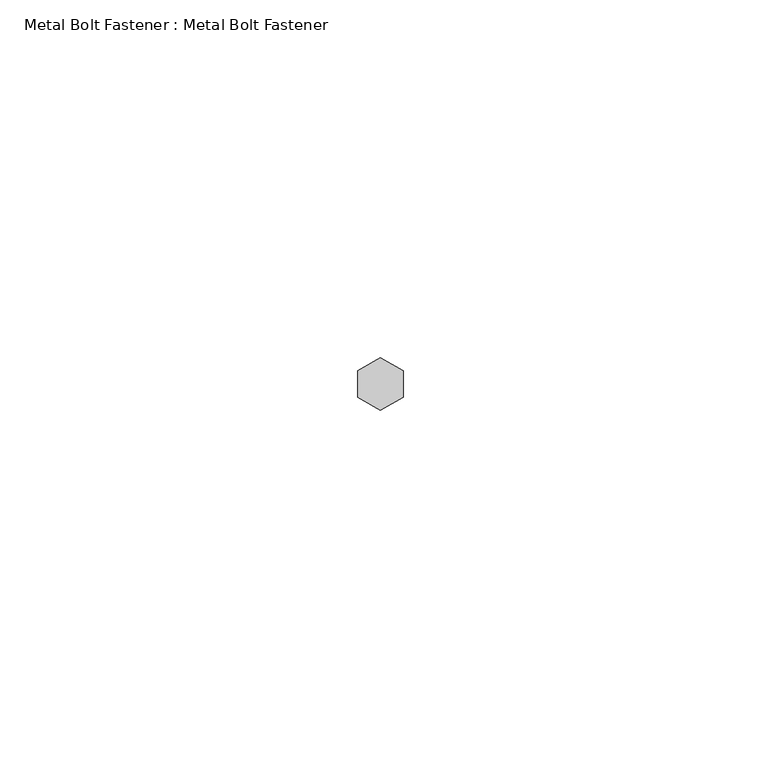
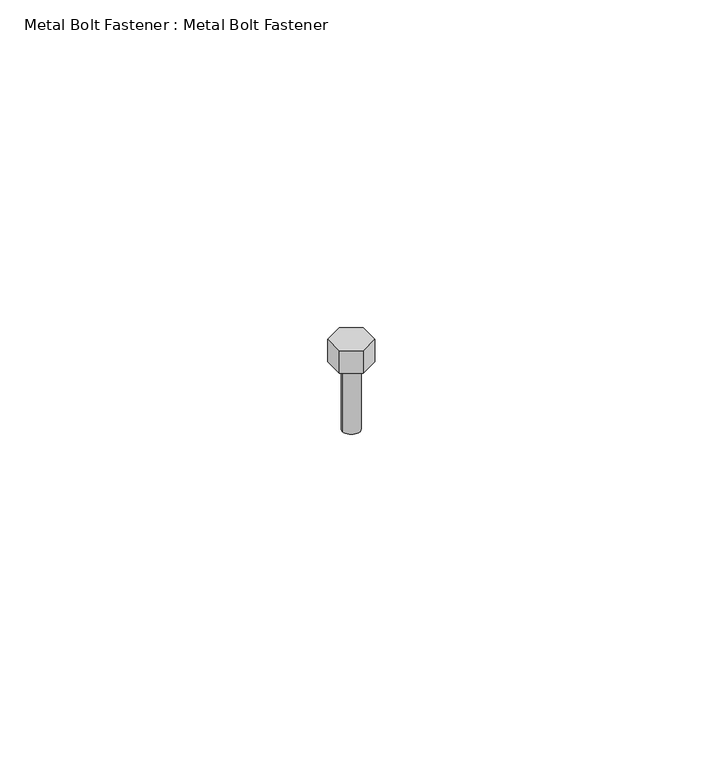
"""IFC4 building model written with IfcOpenShell, lengths in millimetres: proxy geometry, Metal Bolt Fastener : Metal Bolt Fastener."""

from ifc_helpers import new_model, si_unit, frame, origin, origin_with_axes, place, context, project, spatial, polyline, circle_curve, outline, extrude, source, transform, mapped, element, save
from ifc_brep_helpers import plane_surface, cylinder_surface, advanced_brep


def metal_bolt_fastener_metal_bolt_fastener_e4fb09c0(model_context):
    return source(origin(), model_context, "Body", "SolidModel", [
        advanced_brep(
        [(0.0, 0.0, 0.0), (1.5875, 0.0, 0.0), (-1.5875, 0.0, 0.0), (-1.5875, 0.0, -12.7), (1.5875, 0.0, -12.7), (0.0, 0.0, -12.7)],
        [
            (0, 1),
            (1, 2, circle_curve(origin_with_axes(), 1.5875)),
            (2, 0),
            (2, 1, circle_curve(origin_with_axes(), 1.5875)),
            (3, 4, circle_curve(frame((0.0, 0.0, -12.7), z_axis=(0.0, 0.0, -1.0), x_axis=(1.0, 0.0, 0.0)), 1.5875)),
            (4, 5),
            (5, 3),
            (4, 3, circle_curve(frame((0.0, 0.0, -12.7), z_axis=(0.0, 0.0, -1.0), x_axis=(1.0, 0.0, 0.0)), 1.5875)),
            (1, 4),
            (3, 2),
        ],
        [
            plane_surface(origin_with_axes()),
            plane_surface(frame((0.0, 0.0, -12.7), z_axis=(0.0, 0.0, -1.0), x_axis=(1.0, 0.0, 0.0))),
            cylinder_surface(frame((0.0, 0.0, -19.05), z_axis=(0.0, 0.0, 1.0), x_axis=(1.0, 0.0, 0.0)), 1.5875),
        ],
        [
            (0, [[1, 2, 3]]),
            (0, [[-3, 4, -1]]),
            (1, [[5, 6, 7]]),
            (1, [[8, -7, -6]]),
            (2, [[-2, 9, -5, 10]]),
            (2, [[-4, -10, -8, -9]]),
        ],
    ),
        extrude(outline(polyline([(-3.175, 1.8330871), (0.0, 3.6661742), (3.175, 1.8330871), (3.175, -1.8330871), (0.0, -3.6661742), (-3.175, -1.8330871), (-3.175, 1.8330871)])), origin_with_axes(), (0.0, 0.0, 1.0), 4.2333333),
    ])


if __name__ == "__main__":
    model = new_model("IFC4")
    model_context = context("Model", 3, world=origin())
    ifc_project = project(units=[si_unit("LENGTHUNIT", "METRE", prefix="MILLI")], contexts=[model_context])
    site = spatial("IfcSite", under=ifc_project)
    building = spatial("IfcBuilding", under=site)
    placement = place(None, origin())
    metal_bolt_fastener_metal_bolt_fastener_shape = metal_bolt_fastener_metal_bolt_fastener_e4fb09c0(model_context)
    element("IfcBuildingElementProxy", 1, Name="Metal Bolt Fastener : Metal Bolt Fastener", ObjectType="Metal Bolt Fastener : Metal Bolt Fastener", at=placement, inside=building, context=model_context, shape_type="MappedRepresentation", body=[
        mapped(metal_bolt_fastener_metal_bolt_fastener_shape, transform((0.0, 0.0, 0.0), x_axis=(1.0, 0.0, 0.0), y_axis=(0.0, 1.0, 0.0), z_axis=(0.0, 0.0, 1.0))),
    ])
    save(model, "model.ifc")

# Revit data of these elements
# Type "Metal Bolt Fastener : Metal Bolt Fastener"
#   Height = 0' - 0.16667"
#   H2 = 0' - 0 1/2"
#   F3 = 0' - 0 1/16"
#   F2 = 0' - 0 1/8"
#   F = 0' - 0 1/4"
#   Material [instance default] = none
# Element 1 (IfcBuildingElementProxy, "Metal Bolt Fastener : Metal Bolt Fastener")
#   Materials on its faces: "UNISTRUT 1/4\"  FIBERGLASS HEX FLANGED BOLT"
# Materials
#   "UNISTRUT 1/4\"  FIBERGLASS HEX FLANGED BOLT": class "Miscellaneous", colour RGB 236 232 217, transparency 0, Cost = 0
